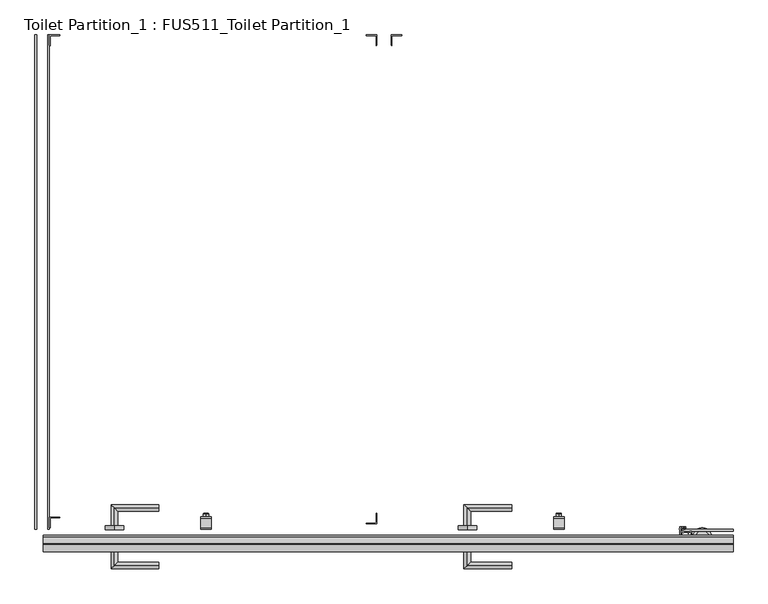
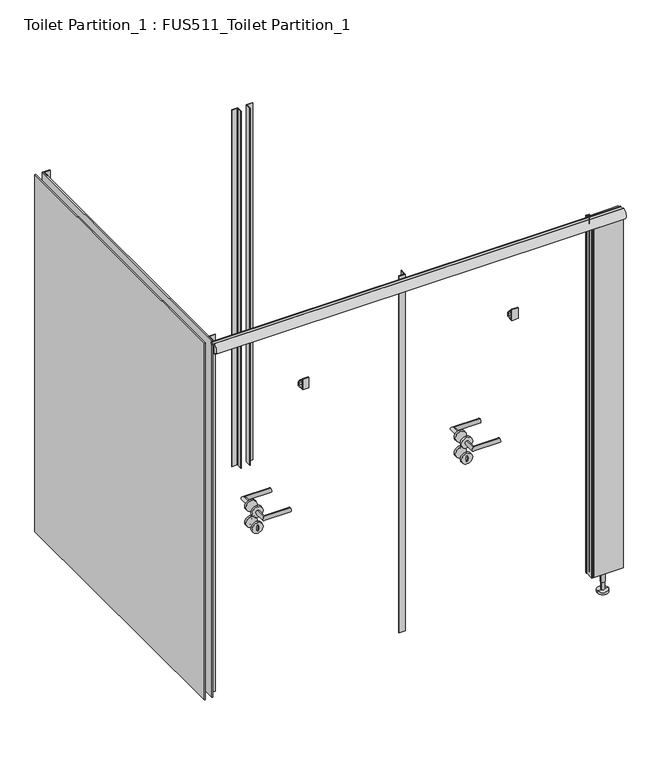
"""IFC4 building model written with IfcOpenShell, lengths in millimetres: furniture geometry, Toilet Partition_1 : FUS511_Toilet Partition_1."""

from ifc_helpers import new_model, si_unit, point, frame, frame_2d, origin, place, context, project, spatial, polyline, circle_curve, ellipse_curve, trimmed, segment, composite_curve, outline, extrude, source, transform, mapped, element, save
from ifc_brep_helpers import plane_surface, cylinder_surface, revolved_surface, extruded_surface, advanced_brep


def toilet_partition_1_fus511_toilet_partition_1_3647186f(model_context):
    return source(origin(), model_context, "Body", "SolidModel", [
        extrude(outline(polyline([(346.5617082, 503.4888254), (346.5617082, 497.0402783), (344.1649522, 497.0402783), (344.1649522, 497.8847941), (345.5746219, 497.8847941), (345.5746219, 501.5146528), (337.5048438, 501.5146528), (341.5634705, 497.0112968), (340.4236814, 497.0112968), (336.3650548, 501.5146528), (332.7425001, 501.5146528), (332.7425001, 454.1345106), (330.7683275, 454.1345106), (330.7683275, 497.4270801), (329.456802, 495.1554513), (328.3170129, 495.1554513), (330.7683275, 499.4012527), (330.7683275, 503.4888254), (346.5617082, 503.4888254)])), frame((0.0, 0.0, 100.0), z_axis=(0.0, 0.0, 1.0), x_axis=(1.0, 0.0, 0.0)), (0.0, 0.0, 1.0), 1800.0),
        extrude(outline(composite_curve([segment(trimmed(circle_curve(frame_2d((341.357373, 496.004016)), 0.789669), [point((341.357373, 495.214347))], [point((340.5677039, 496.004016))], False, "CARTESIAN"), True, "CONTINUOUS"), segment(polyline([(340.5677039, 496.004016), (340.5677039, 496.8402783), (341.715535, 496.8402783)]), True, "CONTINUOUS"), segment(trimmed(circle_curve(frame_2d((341.0726269, 497.4916495)), 0.9152132), [point((341.715535, 496.8402783))], [point((341.665841, 498.1885801))], True, "CARTESIAN"), True, "CONTINUOUS"), segment(trimmed(circle_curve(frame_2d((341.9239046, 498.4917631)), 0.3981417), [point((341.665841, 498.1885801))], [point((341.7737026, 498.8604854))], False, "CARTESIAN"), True, "CONTINUOUS"), segment(trimmed(circle_curve(frame_2d((342.8695936, 496.1702449)), 2.9048875), [point((341.7737026, 498.8604854))], [point((343.9414711, 498.870143))], False, "CARTESIAN"), True, "CONTINUOUS"), segment(trimmed(circle_curve(frame_2d((343.7877156, 498.4828563)), 0.4166915), [point((343.9414711, 498.870143))], [point((344.0660464, 498.1727534))], False, "CARTESIAN"), True, "CONTINUOUS"), segment(trimmed(circle_curve(frame_2d((344.6773667, 497.4916495)), 0.9152132), [point((344.0660464, 498.1727534))], [point((344.0344586, 496.8402783))], True, "CARTESIAN"), True, "CONTINUOUS"), segment(polyline([(344.0344586, 496.8402783), (345.1822897, 496.8402783), (345.1822897, 496.004016)]), True, "CONTINUOUS"), segment(trimmed(circle_curve(frame_2d((344.3926207, 496.004016)), 0.789669), [point((345.1822897, 496.004016))], [point((344.3926207, 495.214347))], False, "CARTESIAN"), True, "CONTINUOUS"), segment(polyline([(344.3926207, 495.214347), (341.357373, 495.214347)]), True, "CONTINUOUS")], self_intersect=False)), frame((0.0, 0.0, 100.0), z_axis=(0.0, 0.0, 1.0), x_axis=(1.0, 0.0, 0.0)), (0.0, 0.0, 1.0), 1800.0),
        advanced_brep(
        [(409.5372607, 474.714347, 104.1461397), (409.5372607, 474.714347, 101.0217555), (378.2934188, 474.714347, 101.0217555), (378.2934188, 474.714347, 104.1461397), (419.9518747, 474.714347, 0.0), (393.9153398, 474.714347, 0.0), (367.8788048, 474.714347, 0.0), (419.9518747, 474.714347, 10.414614), (367.8788048, 474.714347, 10.414614), (401.7263002, 474.714347, 10.414614), (386.1043793, 474.714347, 10.414614), (401.7263002, 474.714347, 52.0730698), (386.1043793, 474.714347, 52.0730698), (404.3299537, 474.714347, 52.0730698), (383.5007258, 474.714347, 52.0730698), (404.3299537, 474.714347, 101.0217555), (383.5007258, 474.714347, 101.0217555), (411.6201835, 474.714347, 104.1461397), (376.210496, 474.714347, 104.1461397), (411.6201835, 474.714347, 110.394908), (376.210496, 474.714347, 110.394908), (393.9153398, 474.714347, 110.394908)],
        [
            (0, 1),
            (1, 2, circle_curve(frame((393.9153398, 474.714347, 101.0217555), z_axis=(0.0, 0.0, 1.0), x_axis=(-1.0, 0.0, 0.0)), 15.6219209)),
            (2, 3),
            (3, 0, circle_curve(frame((393.9153398, 474.714347, 104.1461397), z_axis=(0.0, 0.0, -1.0), x_axis=(-1.0, 0.0, 0.0)), 15.6219209)),
            (2, 1, circle_curve(frame((393.9153398, 474.714347, 101.0217555), z_axis=(0.0, 0.0, 1.0), x_axis=(-1.0, 0.0, 0.0)), 15.6219209)),
            (0, 3, circle_curve(frame((393.9153398, 474.714347, 104.1461397), z_axis=(0.0, 0.0, -1.0), x_axis=(-1.0, 0.0, 0.0)), 15.6219209)),
            (4, 5),
            (5, 6),
            (6, 4, circle_curve(frame((393.9153398, 474.714347, 0.0), z_axis=(0.0, 0.0, -1.0), x_axis=(-1.0, 0.0, 0.0)), 26.0365349)),
            (4, 6, circle_curve(frame((393.9153398, 474.714347, 0.0), z_axis=(0.0, 0.0, -1.0), x_axis=(-1.0, 0.0, 0.0)), 26.0365349)),
            (7, 4),
            (6, 8),
            (8, 7, circle_curve(frame((393.9153398, 474.714347, 10.414614), z_axis=(0.0, 0.0, -1.0), x_axis=(-1.0, 0.0, 0.0)), 26.0365349)),
            (7, 8, circle_curve(frame((393.9153398, 474.714347, 10.414614), z_axis=(0.0, 0.0, -1.0), x_axis=(-1.0, 0.0, 0.0)), 26.0365349)),
            (9, 7),
            (8, 10),
            (10, 9, circle_curve(frame((393.9153398, 474.714347, 10.414614), z_axis=(0.0, 0.0, -1.0), x_axis=(-1.0, 0.0, 0.0)), 7.8109605)),
            (9, 10, circle_curve(frame((393.9153398, 474.714347, 10.414614), z_axis=(0.0, 0.0, -1.0), x_axis=(-1.0, 0.0, 0.0)), 7.8109605)),
            (11, 9),
            (10, 12),
            (12, 11, circle_curve(frame((393.9153398, 474.714347, 52.0730698), z_axis=(0.0, 0.0, -1.0), x_axis=(-1.0, 0.0, 0.0)), 7.8109605)),
            (11, 12, circle_curve(frame((393.9153398, 474.714347, 52.0730698), z_axis=(0.0, 0.0, -1.0), x_axis=(-1.0, 0.0, 0.0)), 7.8109605)),
            (13, 11),
            (12, 14),
            (14, 13, circle_curve(frame((393.9153398, 474.714347, 52.0730698), z_axis=(0.0, 0.0, -1.0), x_axis=(-1.0, 0.0, 0.0)), 10.414614)),
            (13, 14, circle_curve(frame((393.9153398, 474.714347, 52.0730698), z_axis=(0.0, 0.0, -1.0), x_axis=(-1.0, 0.0, 0.0)), 10.414614)),
            (15, 13),
            (14, 16),
            (16, 15, circle_curve(frame((393.9153398, 474.714347, 101.0217555), z_axis=(0.0, 0.0, -1.0), x_axis=(-1.0, 0.0, 0.0)), 10.414614)),
            (15, 16, circle_curve(frame((393.9153398, 474.714347, 101.0217555), z_axis=(0.0, 0.0, -1.0), x_axis=(-1.0, 0.0, 0.0)), 10.414614)),
            (1, 15),
            (16, 2),
            (17, 0),
            (3, 18),
            (18, 17, circle_curve(frame((393.9153398, 474.714347, 104.1461397), z_axis=(0.0, 0.0, -1.0), x_axis=(-1.0, 0.0, 0.0)), 17.7048437)),
            (17, 18, circle_curve(frame((393.9153398, 474.714347, 104.1461397), z_axis=(0.0, 0.0, -1.0), x_axis=(-1.0, 0.0, 0.0)), 17.7048437)),
            (19, 17),
            (18, 20),
            (20, 19, circle_curve(frame((393.9153398, 474.714347, 110.394908), z_axis=(0.0, 0.0, -1.0), x_axis=(-1.0, 0.0, 0.0)), 17.7048437)),
            (19, 20, circle_curve(frame((393.9153398, 474.714347, 110.394908), z_axis=(0.0, 0.0, -1.0), x_axis=(-1.0, 0.0, 0.0)), 17.7048437)),
            (21, 19),
            (20, 21),
        ],
        [
            cylinder_surface(frame((393.9153398, 474.714347, 190.0), z_axis=(0.0, 0.0, 1.0), x_axis=(-1.0, 0.0, 0.0)), 15.6219209),
            plane_surface(frame((393.9153398, 474.714347, 0.0), z_axis=(0.0, 0.0, -1.0), x_axis=(-1.0, 0.0, 0.0))),
            cylinder_surface(frame((393.9153398, 474.714347, 190.0), z_axis=(0.0, 0.0, 1.0), x_axis=(-1.0, 0.0, 0.0)), 26.0365349),
            plane_surface(frame((393.9153398, 474.714347, 10.414614), z_axis=(0.0, 0.0, 1.0), x_axis=(-1.0, 0.0, 0.0))),
            cylinder_surface(frame((393.9153398, 474.714347, 190.0), z_axis=(0.0, 0.0, 1.0), x_axis=(-1.0, 0.0, 0.0)), 7.8109605),
            plane_surface(frame((393.9153398, 474.714347, 52.0730698), z_axis=(0.0, 0.0, -1.0), x_axis=(-1.0, 0.0, 0.0))),
            cylinder_surface(frame((393.9153398, 474.714347, 190.0), z_axis=(0.0, 0.0, 1.0), x_axis=(-1.0, 0.0, 0.0)), 10.414614),
            plane_surface(frame((393.9153398, 474.714347, 101.0217555), z_axis=(0.0, 0.0, -1.0), x_axis=(-1.0, 0.0, 0.0))),
            plane_surface(frame((393.9153398, 474.714347, 104.1461397), z_axis=(0.0, 0.0, -1.0), x_axis=(-1.0, 0.0, 0.0))),
            cylinder_surface(frame((393.9153398, 474.714347, 190.0), z_axis=(0.0, 0.0, 1.0), x_axis=(-1.0, 0.0, 0.0)), 17.7048437),
            plane_surface(frame((393.9153398, 474.714347, 110.394908), z_axis=(0.0, 0.0, 1.0), x_axis=(-1.0, 0.0, 0.0))),
        ],
        [
            (0, [[1, 2, 3, 4]]),
            (0, [[-3, 5, -1, 6]]),
            (1, [[7, 8, 9]]),
            (1, [[-8, -7, 10]]),
            (2, [[11, -9, 12, 13]]),
            (2, [[-12, -10, -11, 14]]),
            (3, [[15, -13, 16, 17]]),
            (3, [[-16, -14, -15, 18]]),
            (4, [[19, -17, 20, 21]]),
            (4, [[-20, -18, -19, 22]]),
            (5, [[23, -21, 24, 25]]),
            (5, [[-24, -22, -23, 26]]),
            (6, [[27, -25, 28, 29]]),
            (6, [[-28, -26, -27, 30]]),
            (7, [[31, -29, 32, -2]]),
            (7, [[-32, -30, -31, -5]]),
            (8, [[33, -4, 34, 35]]),
            (8, [[-34, -6, -33, 36]]),
            (9, [[37, -35, 38, 39]]),
            (9, [[-38, -36, -37, 40]]),
            (10, [[41, -39, 42]]),
            (10, [[-42, -40, -41]]),
        ],
    ),
        extrude(outline(composite_curve([segment(polyline([(363.6512518, 489.5206414), (363.6512518, 459.9080525), (358.7158203, 459.9080525), (358.7158203, 460.8951388), (354.7674751, 460.8951388), (354.7674751, 459.9080525), (341.1950386, 459.9080525)]), True, "CONTINUOUS"), segment(trimmed(circle_curve(frame_2d((340.948267, 460.8637947)), 0.9870863), [point((341.1950386, 459.9080525))], [point((340.7014954, 459.9080525))], True, "CARTESIAN"), True, "CONTINUOUS"), segment(polyline([(340.7014954, 459.9080525), (336.0128355, 459.9080525), (336.0128355, 454.9726211), (335.0257492, 454.9726211)]), True, "CONTINUOUS"), segment(trimmed(circle_curve(frame_2d((335.0257492, 455.9597074)), 0.9870863), [point((335.0257492, 454.9726211))], [point((334.0386629, 455.9597074))], False, "CARTESIAN"), True, "CONTINUOUS"), segment(polyline([(334.0386629, 455.9597074), (334.0386629, 493.4689866)]), True, "CONTINUOUS"), segment(trimmed(circle_curve(frame_2d((335.0257492, 493.4689866)), 0.9870863), [point((334.0386629, 493.4689866))], [point((335.0257492, 494.4560729))], False, "CARTESIAN"), True, "CONTINUOUS"), segment(polyline([(335.0257492, 494.4560729), (336.0128355, 494.4560729), (336.0128355, 489.5206414), (340.7014954, 489.5206414)]), True, "CONTINUOUS"), segment(trimmed(circle_curve(frame_2d((340.948267, 488.5648992)), 0.9870863), [point((340.7014954, 489.5206414))], [point((341.1950386, 489.5206414))], True, "CARTESIAN"), True, "CONTINUOUS"), segment(polyline([(341.1950386, 489.5206414), (354.7674751, 488.5335551), (358.7158203, 488.5335551), (358.7158203, 489.5206414), (363.6512518, 489.5206414)]), True, "CONTINUOUS")], self_intersect=False), holes=[polyline([(360.6899929, 486.5593825), (355.7545614, 486.5593825), (355.7545614, 481.623951), (352.7933025, 481.623951), (352.7933025, 486.5593825), (345.8836985, 486.5593825), (345.8836985, 482.1174942), (344.403069, 482.1174942), (344.403069, 486.5593825), (342.675668, 486.5593825), (342.675668, 484.5852099), (338.7273228, 484.5852099), (338.7273228, 486.5593825), (336.9999218, 486.5593825), (336.9999218, 462.8693114), (338.7273228, 462.8693114), (338.7273228, 464.843484), (342.675668, 464.843484), (342.675668, 462.8693114), (344.403069, 462.8693114), (344.403069, 467.3111998), (345.8836985, 467.3111998), (345.8836985, 462.8693114), (352.7933025, 462.8693114), (352.7933025, 467.8047429), (355.7545614, 467.8047429), (355.7545614, 462.8693114), (360.6899929, 462.8693114), (360.6899929, 486.5593825)])]), frame((0.0, 0.0, 100.0), z_axis=(0.0, 0.0, 1.0), x_axis=(1.0, 0.0, 0.0)), (0.0, 0.0, 1.0), 1800.0),
        extrude(outline(polyline([(481.0128355, 454.214347), (336.0128355, 454.214347), (336.0128355, 459.214347), (481.0128355, 459.214347), (481.0128355, 454.214347)])), frame((0.0, 0.0, 100.0), z_axis=(0.0, 0.0, 1.0), x_axis=(1.0, 0.0, 0.0)), (0.0, 0.0, 1.0), 1800.0),
        extrude(outline(polyline([(481.0128355, 490.214347), (336.0128355, 490.214347), (336.0128355, 495.214347), (481.0128355, 495.214347), (481.0128355, 490.214347)])), frame((0.0, 0.0, 100.0), z_axis=(0.0, 0.0, 1.0), x_axis=(1.0, 0.0, 0.0)), (0.0, 0.0, 1.0), 1800.0),
        extrude(outline(composite_curve([segment(trimmed(circle_curve(frame_2d((-1451.3856706, 1892.2118377)), 1.0008364), [point((-1451.3856706, 1893.2126742))], [point((-1452.386507, 1892.2118377))], True, "CARTESIAN"), True, "CONTINUOUS"), segment(polyline([(-1452.386507, 1892.2118377), (-1452.386507, 1865.1892547), (-1453.3873434, 1865.1892547)]), True, "CONTINUOUS"), segment(trimmed(circle_curve(frame_2d((-1453.3873434, 1866.1900911)), 1.0008364), [point((-1453.3873434, 1865.1892547))], [point((-1454.3881798, 1866.1900911))], False, "CARTESIAN"), True, "CONTINUOUS"), segment(polyline([(-1454.3881798, 1866.1900911), (-1454.3881798, 1895.214347), (-1425.3639239, 1895.214347)]), True, "CONTINUOUS"), segment(trimmed(circle_curve(frame_2d((-1425.3639239, 1894.2135106)), 1.0008364), [point((-1425.3639239, 1895.214347))], [point((-1424.3630875, 1894.2135106))], False, "CARTESIAN"), True, "CONTINUOUS"), segment(polyline([(-1424.3630875, 1894.2135106), (-1424.3630875, 1893.2126742), (-1451.3856706, 1893.2126742)]), True, "CONTINUOUS")], self_intersect=False)), frame((0.0, 0.0, 100.0), z_axis=(0.0, 0.0, 1.0), x_axis=(1.0, 0.0, 0.0)), (0.0, 0.0, 1.0), 1800.0),
        extrude(outline(composite_curve([segment(trimmed(circle_curve(frame_2d((-1451.3856706, 527.0159753)), 1.0008364), [point((-1451.3856706, 528.0168117))], [point((-1452.386507, 527.0159753))], True, "CARTESIAN"), True, "CONTINUOUS"), segment(polyline([(-1452.386507, 527.0159753), (-1452.386507, 499.9933923), (-1453.3873434, 499.9933923)]), True, "CONTINUOUS"), segment(trimmed(circle_curve(frame_2d((-1453.3873434, 500.9942287)), 1.0008364), [point((-1453.3873434, 499.9933923))], [point((-1454.3881798, 500.9942287))], False, "CARTESIAN"), True, "CONTINUOUS"), segment(polyline([(-1454.3881798, 500.9942287), (-1454.3881798, 530.0184846), (-1425.3639239, 530.0184846)]), True, "CONTINUOUS"), segment(trimmed(circle_curve(frame_2d((-1425.3639239, 529.0176481)), 1.0008364), [point((-1425.3639239, 530.0184846))], [point((-1424.3630875, 529.0176481))], False, "CARTESIAN"), True, "CONTINUOUS"), segment(polyline([(-1424.3630875, 529.0176481), (-1424.3630875, 528.0168117), (-1451.3856706, 528.0168117)]), True, "CONTINUOUS")], self_intersect=False)), frame((0.0, 0.0, 100.0), z_axis=(0.0, 0.0, 1.0), x_axis=(1.0, 0.0, 0.0)), (0.0, 0.0, 1.0), 1800.0),
        extrude(outline(polyline([(-1454.3881798, 495.214347), (-1459.3881798, 495.214347), (-1459.3881798, 1895.214347), (-1454.3881798, 1895.214347), (-1454.3881798, 495.214347)])), frame((0.0, 0.0, 100.0), z_axis=(0.0, 0.0, 1.0), x_axis=(1.0, 0.0, 0.0)), (0.0, 0.0, 1.0), 1800.0),
        extrude(outline(polyline([(-1490.3881798, 495.214347), (-1495.3881798, 495.214347), (-1495.3881798, 1895.214347), (-1490.3881798, 1895.214347), (-1490.3881798, 495.214347)])), frame((0.0, 0.0, 100.0), z_axis=(0.0, 0.0, 1.0), x_axis=(1.0, 0.0, 0.0)), (0.0, 0.0, 1.0), 1800.0),
        advanced_brep(
        [(-271.279512, 505.214347, 893.5), (-271.279512, 505.214347, 946.5), (-271.279512, 505.214347, 934.6347495), (-271.279512, 505.214347, 904.6347495), (-271.279512, 495.214347, 893.5), (-271.279512, 495.214347, 946.5), (-271.279512, 499.9019579, 904.6347495), (-271.279512, 499.9019579, 934.6347495)],
        [
            (0, 1, circle_curve(frame((-271.279512, 505.214347, 920.0), z_axis=(0.0, 1.0, 0.0), x_axis=(0.0, 0.0, 1.0)), 26.5)),
            (1, 0, circle_curve(frame((-271.279512, 505.214347, 920.0), z_axis=(0.0, 1.0, 0.0), x_axis=(0.0, 0.0, 1.0)), 26.5)),
            (2, 3, ellipse_curve(frame((-271.279512, 505.214347, 919.6347495), z_axis=(0.0, -1.0, 0.0), x_axis=(0.0, 0.0, 1.0)), 15.0, 5.0)),
            (3, 2, ellipse_curve(frame((-271.279512, 505.214347, 919.6347495), z_axis=(0.0, -1.0, 0.0), x_axis=(0.0, 0.0, 1.0)), 15.0, 5.0)),
            (4, 5, circle_curve(frame((-271.279512, 495.214347, 920.0), z_axis=(0.0, -1.0, 0.0), x_axis=(0.0, 0.0, 1.0)), 26.5)),
            (5, 4, circle_curve(frame((-271.279512, 495.214347, 920.0), z_axis=(0.0, -1.0, 0.0), x_axis=(0.0, 0.0, 1.0)), 26.5)),
            (0, 4),
            (5, 1),
            (6, 7, ellipse_curve(frame((-271.279512, 499.9019579, 919.6347495), z_axis=(0.0, 1.0, 0.0), x_axis=(0.0, 0.0, 1.0)), 15.0, 5.0)),
            (7, 6, ellipse_curve(frame((-271.279512, 499.9019579, 919.6347495), z_axis=(0.0, 1.0, 0.0), x_axis=(0.0, 0.0, 1.0)), 15.0, 5.0)),
            (6, 3),
            (2, 7),
        ],
        [
            plane_surface(frame((-271.279512, 505.214347, 946.5), z_axis=(0.0, 1.0, 0.0), x_axis=(1.0, 0.0, 0.0))),
            plane_surface(frame((-271.279512, 495.214347, 946.5), z_axis=(0.0, -1.0, 0.0), x_axis=(-1.0, 0.0, 0.0))),
            cylinder_surface(frame((-271.279512, 495.214347, 920.0), z_axis=(0.0, 1.0, 0.0), x_axis=(0.0, 0.0, 1.0)), 26.5),
            plane_surface(frame((-271.279512, 499.9019579, 934.6347495), z_axis=(0.0, 1.0, 0.0), x_axis=(-1.0, 0.0, 0.0))),
            extruded_surface(trimmed(ellipse_curve(frame((-271.279512, 499.9019579, 919.6347495), z_axis=(0.0, 1.0, 0.0), x_axis=(0.0, 0.0, 1.0)), 15.0, 5.0), [point((-271.279512, 499.9019579, 904.6347495))], [point((-271.279512, 499.9019579, 934.6347495))], True, "CARTESIAN"), (0.0, -5.312388999999996, 0.0), 5.312388999999996),
            extruded_surface(trimmed(ellipse_curve(frame((-271.279512, 499.9019579, 919.6347495), z_axis=(0.0, 1.0, 0.0), x_axis=(0.0, 0.0, 1.0)), 15.0, 5.0), [point((-271.279512, 499.9019579, 934.6347495))], [point((-271.279512, 499.9019579, 904.6347495))], True, "CARTESIAN"), (0.0, -5.312388999999996, 0.0), 5.312388999999996),
        ],
        [
            (0, [[1, 2], [3, 4]]),
            (1, [[5, 6]]),
            (2, [[-1, 7, -6, 8]]),
            (2, [[-2, -8, -5, -7]]),
            (3, [[9, 10]]),
            (4, [[-9, 11, -3, 12]]),
            (5, [[-10, -12, -4, -11]]),
        ],
    ),
        advanced_brep(
        [(-271.279512, 505.214347, 990.5), (-271.279512, 505.214347, 1009.5), (-271.279512, 555.714347, 990.5), (-271.279512, 555.714347, 1009.5), (-145.779512, 555.714347, 990.5), (-145.779512, 555.714347, 1009.5)],
        [
            (0, 1, circle_curve(frame((-271.279512, 505.214347, 1000.0), z_axis=(0.0, -1.0, 0.0), x_axis=(0.0, 0.0, 1.0)), 9.5)),
            (1, 0, circle_curve(frame((-271.279512, 505.214347, 1000.0), z_axis=(0.0, -1.0, 0.0), x_axis=(0.0, 0.0, 1.0)), 9.5)),
            (0, 2),
            (2, 3, ellipse_curve(frame((-271.279512, 555.714347, 1000.0), z_axis=(-0.7071067811865486, -0.7071067811865465, 0.0), x_axis=(0.7071067811865465, -0.7071067811865485, 0.0)), 13.4350288, 9.5)),
            (3, 1),
            (3, 2, ellipse_curve(frame((-271.279512, 555.714347, 1000.0), z_axis=(-0.7071067811865486, -0.7071067811865465, 0.0), x_axis=(0.7071067811865465, -0.7071067811865485, 0.0)), 13.4350288, 9.5)),
            (4, 5, circle_curve(frame((-145.779512, 555.714347, 1000.0), z_axis=(1.0, 0.0, 0.0), x_axis=(0.0, 0.0, 1.0)), 9.5)),
            (5, 4, circle_curve(frame((-145.779512, 555.714347, 1000.0), z_axis=(1.0, 0.0, 0.0), x_axis=(0.0, 0.0, 1.0)), 9.5)),
            (2, 4),
            (5, 3),
        ],
        [
            plane_surface(frame((-280.779512, 505.214347, 1000.0), z_axis=(0.0, -1.0, 0.0), x_axis=(0.0, 0.0, 1.0))),
            cylinder_surface(frame((-271.279512, 505.214347, 1000.0), z_axis=(0.0, -1.0, 0.0), x_axis=(0.0, 0.0, 1.0)), 9.5),
            plane_surface(frame((-145.779512, 565.214347, 1000.0), z_axis=(1.0, 0.0, 0.0), x_axis=(0.0, 0.0, 1.0))),
            cylinder_surface(frame((-280.779512, 555.714347, 1000.0), z_axis=(-1.0, 0.0, 0.0), x_axis=(0.0, 0.0, 1.0)), 9.5),
        ],
        [
            (0, [[1, 2]]),
            (1, [[-1, 3, 4, 5]]),
            (1, [[-2, -5, 6, -3]]),
            (2, [[7, 8]]),
            (3, [[-4, 9, -8, 10]]),
            (3, [[-6, -10, -7, -9]]),
        ],
    ),
        extrude(outline(composite_curve([segment(trimmed(circle_curve(frame_2d((1000.0, -271.279512)), 26.5), [point((973.5, -271.279512))], [point((1026.5, -271.279512))], False, "CARTESIAN"), True, "CONTINUOUS"), segment(trimmed(circle_curve(frame_2d((1000.0, -271.279512)), 26.5), [point((1026.5, -271.279512))], [point((973.5, -271.279512))], False, "CARTESIAN"), True, "CONTINUOUS")], self_intersect=False)), frame((0.0, 495.214347, 0.0), z_axis=(0.0, 1.0, 0.0), x_axis=(0.0, 0.0, 1.0)), (0.0, 0.0, 1.0), 10.0),
        advanced_brep(
        [(-1270.2108466, 505.214347, 893.5), (-1270.2108466, 505.214347, 946.5), (-1270.2108466, 505.214347, 934.6347495), (-1270.2108466, 505.214347, 904.6347495), (-1270.2108466, 495.214347, 893.5), (-1270.2108466, 495.214347, 946.5), (-1270.2108466, 499.9019579, 904.6347495), (-1270.2108466, 499.9019579, 934.6347495)],
        [
            (0, 1, circle_curve(frame((-1270.2108466, 505.214347, 920.0), z_axis=(0.0, 1.0, 0.0), x_axis=(0.0, 0.0, 1.0)), 26.5)),
            (1, 0, circle_curve(frame((-1270.2108466, 505.214347, 920.0), z_axis=(0.0, 1.0, 0.0), x_axis=(0.0, 0.0, 1.0)), 26.5)),
            (2, 3, ellipse_curve(frame((-1270.2108466, 505.214347, 919.6347495), z_axis=(0.0, -1.0, 0.0), x_axis=(0.0, 0.0, 1.0)), 15.0, 5.0)),
            (3, 2, ellipse_curve(frame((-1270.2108466, 505.214347, 919.6347495), z_axis=(0.0, -1.0, 0.0), x_axis=(0.0, 0.0, 1.0)), 15.0, 5.0)),
            (4, 5, circle_curve(frame((-1270.2108466, 495.214347, 920.0), z_axis=(0.0, -1.0, 0.0), x_axis=(0.0, 0.0, 1.0)), 26.5)),
            (5, 4, circle_curve(frame((-1270.2108466, 495.214347, 920.0), z_axis=(0.0, -1.0, 0.0), x_axis=(0.0, 0.0, 1.0)), 26.5)),
            (0, 4),
            (5, 1),
            (6, 7, ellipse_curve(frame((-1270.2108466, 499.9019579, 919.6347495), z_axis=(0.0, 1.0, 0.0), x_axis=(0.0, 0.0, 1.0)), 15.0, 5.0)),
            (7, 6, ellipse_curve(frame((-1270.2108466, 499.9019579, 919.6347495), z_axis=(0.0, 1.0, 0.0), x_axis=(0.0, 0.0, 1.0)), 15.0, 5.0)),
            (6, 3),
            (2, 7),
        ],
        [
            plane_surface(frame((-1270.2108466, 505.214347, 946.5), z_axis=(0.0, 1.0, 0.0), x_axis=(1.0, 0.0, 0.0))),
            plane_surface(frame((-1270.2108466, 495.214347, 946.5), z_axis=(0.0, -1.0, 0.0), x_axis=(-1.0, 0.0, 0.0))),
            cylinder_surface(frame((-1270.2108466, 495.214347, 920.0), z_axis=(0.0, 1.0, 0.0), x_axis=(0.0, 0.0, 1.0)), 26.5),
            plane_surface(frame((-1270.2108466, 499.9019579, 934.6347495), z_axis=(0.0, 1.0, 0.0), x_axis=(-1.0, 0.0, 0.0))),
            extruded_surface(trimmed(ellipse_curve(frame((-1270.2108466, 499.9019579, 919.6347495), z_axis=(0.0, 1.0, 0.0), x_axis=(0.0, 0.0, 1.0)), 15.0, 5.0), [point((-1270.2108466, 499.9019579, 904.6347495))], [point((-1270.2108466, 499.9019579, 934.6347495))], True, "CARTESIAN"), (0.0, -5.312388999999996, 0.0), 5.312388999999996),
            extruded_surface(trimmed(ellipse_curve(frame((-1270.2108466, 499.9019579, 919.6347495), z_axis=(0.0, 1.0, 0.0), x_axis=(0.0, 0.0, 1.0)), 15.0, 5.0), [point((-1270.2108466, 499.9019579, 934.6347495))], [point((-1270.2108466, 499.9019579, 904.6347495))], True, "CARTESIAN"), (0.0, -5.312388999999996, 0.0), 5.312388999999996),
        ],
        [
            (0, [[1, 2], [3, 4]]),
            (1, [[5, 6]]),
            (2, [[-1, 7, -6, 8]]),
            (2, [[-2, -8, -5, -7]]),
            (3, [[9, 10]]),
            (4, [[-9, 11, -3, 12]]),
            (5, [[-10, -12, -4, -11]]),
        ],
    ),
        advanced_brep(
        [(-1270.2108466, 505.214347, 990.5), (-1270.2108466, 505.214347, 1009.5), (-1270.2108466, 555.714347, 990.5), (-1270.2108466, 555.714347, 1009.5), (-1144.7108466, 555.714347, 990.5), (-1144.7108466, 555.714347, 1009.5)],
        [
            (0, 1, circle_curve(frame((-1270.2108466, 505.214347, 1000.0), z_axis=(0.0, -1.0, 0.0), x_axis=(0.0, 0.0, 1.0)), 9.5)),
            (1, 0, circle_curve(frame((-1270.2108466, 505.214347, 1000.0), z_axis=(0.0, -1.0, 0.0), x_axis=(0.0, 0.0, 1.0)), 9.5)),
            (0, 2),
            (2, 3, ellipse_curve(frame((-1270.2108466, 555.714347, 1000.0), z_axis=(-0.7071067811865486, -0.7071067811865465, 0.0), x_axis=(0.7071067811865465, -0.7071067811865485, 0.0)), 13.4350288, 9.5)),
            (3, 1),
            (3, 2, ellipse_curve(frame((-1270.2108466, 555.714347, 1000.0), z_axis=(-0.7071067811865486, -0.7071067811865465, 0.0), x_axis=(0.7071067811865465, -0.7071067811865485, 0.0)), 13.4350288, 9.5)),
            (4, 5, circle_curve(frame((-1144.7108466, 555.714347, 1000.0), z_axis=(1.0, 0.0, 0.0), x_axis=(0.0, 0.0, 1.0)), 9.5)),
            (5, 4, circle_curve(frame((-1144.7108466, 555.714347, 1000.0), z_axis=(1.0, 0.0, 0.0), x_axis=(0.0, 0.0, 1.0)), 9.5)),
            (2, 4),
            (5, 3),
        ],
        [
            plane_surface(frame((-1279.7108466, 505.214347, 1000.0), z_axis=(0.0, -1.0, 0.0), x_axis=(0.0, 0.0, 1.0))),
            cylinder_surface(frame((-1270.2108466, 505.214347, 1000.0), z_axis=(0.0, -1.0, 0.0), x_axis=(0.0, 0.0, 1.0)), 9.5),
            plane_surface(frame((-1144.7108466, 565.214347, 1000.0), z_axis=(1.0, 0.0, 0.0), x_axis=(0.0, 0.0, 1.0))),
            cylinder_surface(frame((-1279.7108466, 555.714347, 1000.0), z_axis=(-1.0, 0.0, 0.0), x_axis=(0.0, 0.0, 1.0)), 9.5),
        ],
        [
            (0, [[1, 2]]),
            (1, [[-1, 3, 4, 5]]),
            (1, [[-2, -5, 6, -3]]),
            (2, [[7, 8]]),
            (3, [[-4, 9, -8, 10]]),
            (3, [[-6, -10, -7, -9]]),
        ],
    ),
        extrude(outline(composite_curve([segment(trimmed(circle_curve(frame_2d((1000.0, -1270.2108466)), 26.5), [point((973.5, -1270.2108466))], [point((1026.5, -1270.2108466))], False, "CARTESIAN"), True, "CONTINUOUS"), segment(trimmed(circle_curve(frame_2d((1000.0, -1270.2108466)), 26.5), [point((1026.5, -1270.2108466))], [point((973.5, -1270.2108466))], False, "CARTESIAN"), True, "CONTINUOUS")], self_intersect=False)), frame((0.0, 495.214347, 0.0), z_axis=(0.0, 1.0, 0.0), x_axis=(0.0, 0.0, 1.0)), (0.0, 0.0, 1.0), 10.0),
        advanced_brep(
        [(-271.279512, 444.214347, 893.5), (-271.279512, 444.214347, 946.5), (-271.279512, 444.214347, 934.6347495), (-271.279512, 444.214347, 904.6347495), (-271.279512, 454.214347, 893.5), (-271.279512, 454.214347, 946.5), (-271.279512, 449.526736, 904.6347495), (-271.279512, 449.526736, 934.6347495)],
        [
            (0, 1, circle_curve(frame((-271.279512, 444.214347, 920.0), z_axis=(0.0, -1.0, 0.0), x_axis=(0.0, 0.0, 1.0)), 26.5)),
            (1, 0, circle_curve(frame((-271.279512, 444.214347, 920.0), z_axis=(0.0, -1.0, 0.0), x_axis=(0.0, 0.0, 1.0)), 26.5)),
            (2, 3, ellipse_curve(frame((-271.279512, 444.214347, 919.6347495), z_axis=(0.0, 1.0, 0.0), x_axis=(0.0, 0.0, 1.0)), 15.0, 5.0)),
            (3, 2, ellipse_curve(frame((-271.279512, 444.214347, 919.6347495), z_axis=(0.0, 1.0, 0.0), x_axis=(0.0, 0.0, 1.0)), 15.0, 5.0)),
            (4, 5, circle_curve(frame((-271.279512, 454.214347, 920.0), z_axis=(0.0, 1.0, 0.0), x_axis=(0.0, 0.0, 1.0)), 26.5)),
            (5, 4, circle_curve(frame((-271.279512, 454.214347, 920.0), z_axis=(0.0, 1.0, 0.0), x_axis=(0.0, 0.0, 1.0)), 26.5)),
            (1, 5),
            (4, 0),
            (6, 7, ellipse_curve(frame((-271.279512, 449.526736, 919.6347495), z_axis=(0.0, -1.0, 0.0), x_axis=(0.0, 0.0, 1.0)), 15.0, 5.0)),
            (7, 6, ellipse_curve(frame((-271.279512, 449.526736, 919.6347495), z_axis=(0.0, -1.0, 0.0), x_axis=(0.0, 0.0, 1.0)), 15.0, 5.0)),
            (7, 2),
            (3, 6),
        ],
        [
            plane_surface(frame((-271.279512, 444.214347, 946.5), z_axis=(0.0, -1.0, 0.0), x_axis=(1.0, 0.0, 0.0))),
            plane_surface(frame((-271.279512, 454.214347, 946.5), z_axis=(0.0, 1.0, 0.0), x_axis=(-1.0, 0.0, 0.0))),
            cylinder_surface(frame((-271.279512, 454.214347, 920.0), z_axis=(0.0, -1.0, 0.0), x_axis=(0.0, 0.0, 1.0)), 26.5),
            plane_surface(frame((-271.279512, 449.526736, 934.6347495), z_axis=(0.0, -1.0, 0.0), x_axis=(-1.0, 0.0, 0.0))),
            extruded_surface(trimmed(ellipse_curve(frame((-271.279512, 454.8391251, 919.6347495), z_axis=(0.0, 1.0, 0.0), x_axis=(0.0, 0.0, 1.0)), 15.0, 5.0), [point((-271.279512, 454.8391251, 904.6347495))], [point((-271.279512, 454.8391251, 934.6347495))], True, "CARTESIAN"), (0.0, -5.312389099999962, 0.0), 5.312389099999962),
            extruded_surface(trimmed(ellipse_curve(frame((-271.279512, 454.8391251, 919.6347495), z_axis=(0.0, 1.0, 0.0), x_axis=(0.0, 0.0, 1.0)), 15.0, 5.0), [point((-271.279512, 454.8391251, 934.6347495))], [point((-271.279512, 454.8391251, 904.6347495))], True, "CARTESIAN"), (0.0, -5.312389099999962, 0.0), 5.312389099999962),
        ],
        [
            (0, [[1, 2], [3, 4]]),
            (1, [[5, 6]]),
            (2, [[7, -5, 8, -2]]),
            (2, [[-8, -6, -7, -1]]),
            (3, [[9, 10]]),
            (4, [[11, -4, 12, -10]]),
            (5, [[-12, -3, -11, -9]]),
        ],
    ),
        advanced_brep(
        [(-271.279512, 444.214347, 990.5), (-271.279512, 444.214347, 1009.5), (-271.279512, 393.714347, 1009.5), (-271.279512, 393.714347, 990.5), (-145.779512, 393.714347, 990.5), (-145.779512, 393.714347, 1009.5)],
        [
            (0, 1, circle_curve(frame((-271.279512, 444.214347, 1000.0), z_axis=(0.0, 1.0, 0.0), x_axis=(0.0, 0.0, 1.0)), 9.5)),
            (1, 0, circle_curve(frame((-271.279512, 444.214347, 1000.0), z_axis=(0.0, 1.0, 0.0), x_axis=(0.0, 0.0, 1.0)), 9.5)),
            (1, 2),
            (2, 3, ellipse_curve(frame((-271.279512, 393.714347, 1000.0), z_axis=(-0.7071067811865486, 0.7071067811865465, 0.0), x_axis=(0.7071067811865465, 0.7071067811865485, 0.0)), 13.4350288, 9.5)),
            (3, 0),
            (3, 2, ellipse_curve(frame((-271.279512, 393.714347, 1000.0), z_axis=(-0.7071067811865486, 0.7071067811865465, 0.0), x_axis=(0.7071067811865465, 0.7071067811865485, 0.0)), 13.4350288, 9.5)),
            (4, 5, circle_curve(frame((-145.779512, 393.714347, 1000.0), z_axis=(1.0, 0.0, 0.0), x_axis=(0.0, 0.0, 1.0)), 9.5)),
            (5, 4, circle_curve(frame((-145.779512, 393.714347, 1000.0), z_axis=(1.0, 0.0, 0.0), x_axis=(0.0, 0.0, 1.0)), 9.5)),
            (2, 5),
            (4, 3),
        ],
        [
            plane_surface(frame((-280.779512, 444.214347, 1000.0), z_axis=(0.0, 1.0, 0.0), x_axis=(0.0, 0.0, 1.0))),
            cylinder_surface(frame((-271.279512, 444.214347, 1000.0), z_axis=(0.0, 1.0, 0.0), x_axis=(0.0, 0.0, 1.0)), 9.5),
            plane_surface(frame((-145.779512, 384.214347, 1000.0), z_axis=(1.0, 0.0, 0.0), x_axis=(0.0, 0.0, 1.0))),
            cylinder_surface(frame((-280.779512, 393.714347, 1000.0), z_axis=(-1.0, 0.0, 0.0), x_axis=(0.0, 0.0, 1.0)), 9.5),
        ],
        [
            (0, [[1, 2]]),
            (1, [[3, 4, 5, -2]]),
            (1, [[-5, 6, -3, -1]]),
            (2, [[7, 8]]),
            (3, [[9, -7, 10, -4]]),
            (3, [[-10, -8, -9, -6]]),
        ],
    ),
        extrude(outline(composite_curve([segment(trimmed(circle_curve(frame_2d((1000.0, -271.279512)), 26.5), [point((973.5, -271.279512))], [point((1026.5, -271.279512))], False, "CARTESIAN"), True, "CONTINUOUS"), segment(trimmed(circle_curve(frame_2d((1000.0, -271.279512)), 26.5), [point((1026.5, -271.279512))], [point((973.5, -271.279512))], False, "CARTESIAN"), True, "CONTINUOUS")], self_intersect=False)), frame((0.0, 444.214347, 0.0), z_axis=(0.0, 1.0, 0.0), x_axis=(0.0, 0.0, 1.0)), (0.0, 0.0, 1.0), 10.0),
        advanced_brep(
        [(-1270.2108466, 444.214347, 893.5), (-1270.2108466, 444.214347, 946.5), (-1270.2108466, 444.214347, 934.6347495), (-1270.2108466, 444.214347, 904.6347495), (-1270.2108466, 454.214347, 893.5), (-1270.2108466, 454.214347, 946.5), (-1270.2108466, 449.526736, 904.6347495), (-1270.2108466, 449.526736, 934.6347495)],
        [
            (0, 1, circle_curve(frame((-1270.2108466, 444.214347, 920.0), z_axis=(0.0, -1.0, 0.0), x_axis=(0.0, 0.0, 1.0)), 26.5)),
            (1, 0, circle_curve(frame((-1270.2108466, 444.214347, 920.0), z_axis=(0.0, -1.0, 0.0), x_axis=(0.0, 0.0, 1.0)), 26.5)),
            (2, 3, ellipse_curve(frame((-1270.2108466, 444.214347, 919.6347495), z_axis=(0.0, 1.0, 0.0), x_axis=(0.0, 0.0, 1.0)), 15.0, 5.0)),
            (3, 2, ellipse_curve(frame((-1270.2108466, 444.214347, 919.6347495), z_axis=(0.0, 1.0, 0.0), x_axis=(0.0, 0.0, 1.0)), 15.0, 5.0)),
            (4, 5, circle_curve(frame((-1270.2108466, 454.214347, 920.0), z_axis=(0.0, 1.0, 0.0), x_axis=(0.0, 0.0, 1.0)), 26.5)),
            (5, 4, circle_curve(frame((-1270.2108466, 454.214347, 920.0), z_axis=(0.0, 1.0, 0.0), x_axis=(0.0, 0.0, 1.0)), 26.5)),
            (1, 5),
            (4, 0),
            (6, 7, ellipse_curve(frame((-1270.2108466, 449.526736, 919.6347495), z_axis=(0.0, -1.0, 0.0), x_axis=(0.0, 0.0, 1.0)), 15.0, 5.0)),
            (7, 6, ellipse_curve(frame((-1270.2108466, 449.526736, 919.6347495), z_axis=(0.0, -1.0, 0.0), x_axis=(0.0, 0.0, 1.0)), 15.0, 5.0)),
            (7, 2),
            (3, 6),
        ],
        [
            plane_surface(frame((-1270.2108466, 444.214347, 946.5), z_axis=(0.0, -1.0, 0.0), x_axis=(1.0, 0.0, 0.0))),
            plane_surface(frame((-1270.2108466, 454.214347, 946.5), z_axis=(0.0, 1.0, 0.0), x_axis=(-1.0, 0.0, 0.0))),
            cylinder_surface(frame((-1270.2108466, 454.214347, 920.0), z_axis=(0.0, -1.0, 0.0), x_axis=(0.0, 0.0, 1.0)), 26.5),
            plane_surface(frame((-1270.2108466, 449.526736, 934.6347495), z_axis=(0.0, -1.0, 0.0), x_axis=(-1.0, 0.0, 0.0))),
            extruded_surface(trimmed(ellipse_curve(frame((-1270.2108466, 454.8391251, 919.6347495), z_axis=(0.0, 1.0, 0.0), x_axis=(0.0, 0.0, 1.0)), 15.0, 5.0), [point((-1270.2108466, 454.8391251, 904.6347495))], [point((-1270.2108466, 454.8391251, 934.6347495))], True, "CARTESIAN"), (0.0, -5.312389099999962, 0.0), 5.312389099999962),
            extruded_surface(trimmed(ellipse_curve(frame((-1270.2108466, 454.8391251, 919.6347495), z_axis=(0.0, 1.0, 0.0), x_axis=(0.0, 0.0, 1.0)), 15.0, 5.0), [point((-1270.2108466, 454.8391251, 934.6347495))], [point((-1270.2108466, 454.8391251, 904.6347495))], True, "CARTESIAN"), (0.0, -5.312389099999962, 0.0), 5.312389099999962),
        ],
        [
            (0, [[1, 2], [3, 4]]),
            (1, [[5, 6]]),
            (2, [[7, -5, 8, -2]]),
            (2, [[-8, -6, -7, -1]]),
            (3, [[9, 10]]),
            (4, [[11, -4, 12, -10]]),
            (5, [[-12, -3, -11, -9]]),
        ],
    ),
        advanced_brep(
        [(-1270.2108466, 444.214347, 990.5), (-1270.2108466, 444.214347, 1009.5), (-1270.2108466, 393.714347, 1009.5), (-1270.2108466, 393.714347, 990.5), (-1144.7108466, 393.714347, 990.5), (-1144.7108466, 393.714347, 1009.5)],
        [
            (0, 1, circle_curve(frame((-1270.2108466, 444.214347, 1000.0), z_axis=(0.0, 1.0, 0.0), x_axis=(0.0, 0.0, 1.0)), 9.5)),
            (1, 0, circle_curve(frame((-1270.2108466, 444.214347, 1000.0), z_axis=(0.0, 1.0, 0.0), x_axis=(0.0, 0.0, 1.0)), 9.5)),
            (1, 2),
            (2, 3, ellipse_curve(frame((-1270.2108466, 393.714347, 1000.0), z_axis=(-0.7071067811865486, 0.7071067811865465, 0.0), x_axis=(0.7071067811865465, 0.7071067811865485, 0.0)), 13.4350288, 9.5)),
            (3, 0),
            (3, 2, ellipse_curve(frame((-1270.2108466, 393.714347, 1000.0), z_axis=(-0.7071067811865486, 0.7071067811865465, 0.0), x_axis=(0.7071067811865465, 0.7071067811865485, 0.0)), 13.4350288, 9.5)),
            (4, 5, circle_curve(frame((-1144.7108466, 393.714347, 1000.0), z_axis=(1.0, 0.0, 0.0), x_axis=(0.0, 0.0, 1.0)), 9.5)),
            (5, 4, circle_curve(frame((-1144.7108466, 393.714347, 1000.0), z_axis=(1.0, 0.0, 0.0), x_axis=(0.0, 0.0, 1.0)), 9.5)),
            (2, 5),
            (4, 3),
        ],
        [
            plane_surface(frame((-1279.7108466, 444.214347, 1000.0), z_axis=(0.0, 1.0, 0.0), x_axis=(0.0, 0.0, 1.0))),
            cylinder_surface(frame((-1270.2108466, 444.214347, 1000.0), z_axis=(0.0, 1.0, 0.0), x_axis=(0.0, 0.0, 1.0)), 9.5),
            plane_surface(frame((-1144.7108466, 384.214347, 1000.0), z_axis=(1.0, 0.0, 0.0), x_axis=(0.0, 0.0, 1.0))),
            cylinder_surface(frame((-1279.7108466, 393.714347, 1000.0), z_axis=(-1.0, 0.0, 0.0), x_axis=(0.0, 0.0, 1.0)), 9.5),
        ],
        [
            (0, [[1, 2]]),
            (1, [[3, 4, 5, -2]]),
            (1, [[-5, 6, -3, -1]]),
            (2, [[7, 8]]),
            (3, [[9, -7, 10, -4]]),
            (3, [[-10, -8, -9, -6]]),
        ],
    ),
        extrude(outline(composite_curve([segment(trimmed(circle_curve(frame_2d((1000.0, -1270.2108466)), 26.5), [point((973.5, -1270.2108466))], [point((1026.5, -1270.2108466))], False, "CARTESIAN"), True, "CONTINUOUS"), segment(trimmed(circle_curve(frame_2d((1000.0, -1270.2108466)), 26.5), [point((1026.5, -1270.2108466))], [point((973.5, -1270.2108466))], False, "CARTESIAN"), True, "CONTINUOUS")], self_intersect=False)), frame((0.0, 444.214347, 0.0), z_axis=(0.0, 1.0, 0.0), x_axis=(0.0, 0.0, 1.0)), (0.0, 0.0, 1.0), 10.0),
        extrude(outline(composite_curve([segment(trimmed(circle_curve(frame_2d((458.4868618, 1888.0268612)), 26.5042707), [point((454.214347, 1861.869224))], [point((453.0212869, 1913.9614685))], False, "CARTESIAN"), True, "CONTINUOUS"), segment(trimmed(circle_curve(frame_2d((453.1556919, 1912.91138)), 1.058655), [point((453.0212869, 1913.9614685))], [point((454.214347, 1912.91138))], False, "CARTESIAN"), True, "CONTINUOUS"), segment(polyline([(454.214347, 1912.91138), (454.214347, 1909.5278954), (474.6592543, 1909.5278954)]), True, "CONTINUOUS"), segment(trimmed(circle_curve(frame_2d((474.2293597, 1904.6828737)), 4.8640564), [point((474.6592543, 1909.5278954))], [point((479.0927404, 1904.7639477))], False, "CARTESIAN"), True, "CONTINUOUS"), segment(trimmed(circle_curve(frame_2d((474.2293597, 1904.8450217)), 4.8640564), [point((479.0927404, 1904.7639477))], [point((473.7994652, 1900.0))], False, "CARTESIAN"), True, "CONTINUOUS"), segment(polyline([(473.7994652, 1900.0), (454.214347, 1900.0), (454.214347, 1861.869224)]), True, "CONTINUOUS")], self_intersect=False), holes=[composite_curve([segment(polyline([(473.939812, 1907.9461271), (455.8017383, 1907.9399126), (455.8017383, 1901.5879827), (473.9398142, 1901.5817682)]), True, "CONTINUOUS"), segment(trimmed(circle_curve(frame_2d((473.9325063, 1904.7639477)), 3.1821878), [point((473.9398142, 1901.5817682))], [point((473.939812, 1907.9461271))], True, "CARTESIAN"), True, "CONTINUOUS")], self_intersect=False), composite_curve([segment(trimmed(circle_curve(frame_2d((457.6658618, 1888.0268612)), 24.6245189), [point((452.6263644, 1912.1301887))], [point((452.6263644, 1863.9235337))], True, "CARTESIAN"), True, "CONTINUOUS"), segment(polyline([(452.6263644, 1863.9235337), (452.6263644, 1912.1301887)]), True, "CONTINUOUS")], self_intersect=False)]), frame((-1471.8881798, 0.0, 0.0), z_axis=(1.0, 0.0, 0.0), x_axis=(0.0, 1.0, 0.0)), (0.0, 0.0, 1.0), 1953.0),
        extrude(outline(composite_curve([segment(polyline([(499.2367016, 1553.2961991), (499.2367016, 1504.0), (527.3931841, 1504.0), (527.3931841, 1516.0894186)]), True, "CONTINUOUS"), segment(trimmed(circle_curve(frame_2d((531.4155388, 1516.0894186)), 4.0223546), [point((527.3931841, 1516.0894186))], [point((531.4155388, 1520.1117732))], False, "CARTESIAN"), True, "CONTINUOUS"), segment(polyline([(531.4155388, 1520.1117732), (531.4155388, 1500.0), (499.2367016, 1500.0), (495.214347, 1500.0), (495.214347, 1553.2961991), (499.2367016, 1553.2961991)]), True, "CONTINUOUS")], self_intersect=False)), frame((-1026.1694992, 0.0, 0.0), z_axis=(1.0, 0.0, 0.0), x_axis=(0.0, 1.0, 0.0)), (0.0, 0.0, 1.0), 30.0),
        advanced_brep(
        [(-1011.1694992, 531.4155388, 1510.5586809), (-1011.1694992, 531.4155388, 1518.1005959), (-1011.1694992, 531.4155388, 1503.016766), (-1011.1694992, 541.4714254, 1506.033532), (-1011.1694992, 541.4714254, 1515.0838299), (-1011.1694992, 541.4714254, 1510.5586809), (-1011.1694992, 539.4602481, 1503.016766), (-1011.1694992, 539.4602481, 1518.1005959)],
        [
            (0, 1),
            (1, 2, circle_curve(frame((-1011.1694992, 531.4155388, 1510.5586809), z_axis=(0.0, -1.0, 0.0), x_axis=(0.0, 0.0, 1.0)), 7.541915)),
            (2, 0),
            (2, 1, circle_curve(frame((-1011.1694992, 531.4155388, 1510.5586809), z_axis=(0.0, -1.0, 0.0), x_axis=(0.0, 0.0, 1.0)), 7.541915)),
            (3, 4, circle_curve(frame((-1011.1694992, 541.4714254, 1510.5586809), z_axis=(0.0, 1.0, 0.0), x_axis=(0.0, 0.0, 1.0)), 4.525149)),
            (4, 5),
            (5, 3),
            (4, 3, circle_curve(frame((-1011.1694992, 541.4714254, 1510.5586809), z_axis=(0.0, 1.0, 0.0), x_axis=(0.0, 0.0, 1.0)), 4.525149)),
            (6, 7, circle_curve(frame((-1011.1694992, 539.4602481, 1510.5586809), z_axis=(0.0, 1.0, 0.0), x_axis=(0.0, 0.0, 1.0)), 7.541915)),
            (7, 4, circle_curve(frame((-1011.1694992, 538.111954, 1515.0229578), z_axis=(-1.0, 0.0, 0.0), x_axis=(0.0, 0.0, -1.0)), 3.3600228)),
            (3, 6, circle_curve(frame((-1011.1694992, 538.111954, 1506.0944041), z_axis=(-1.0, 0.0, 0.0), x_axis=(0.0, 0.0, 1.0)), 3.3600228)),
            (7, 6, circle_curve(frame((-1011.1694992, 539.4602481, 1510.5586809), z_axis=(0.0, 1.0, 0.0), x_axis=(0.0, 0.0, 1.0)), 7.541915)),
            (1, 7),
            (6, 2),
        ],
        [
            plane_surface(frame((-1011.1694992, 531.4155388, 1510.5586809), z_axis=(0.0, -1.0, 0.0), x_axis=(0.0, 0.0, 1.0))),
            plane_surface(frame((-1011.1694992, 541.4714254, 1510.5586809), z_axis=(0.0, 1.0, 0.0), x_axis=(0.0, 0.0, 1.0))),
            revolved_surface(trimmed(ellipse_curve(frame((-1011.1694992, 538.111954, 1515.0229578), z_axis=(1.0, 0.0, 0.0), x_axis=(0.0, 0.0, -1.0)), 3.3600228, 3.3600228), [point((-1011.1694992, 541.4714254, 1515.0838299))], [point((-1011.1694992, 539.4602481, 1518.1005959))], True, "CARTESIAN"), (-1011.1694992, 521.4714254, 1510.5586809), (0.0, -1.0, 0.0)),
            cylinder_surface(frame((-1011.1694992, 521.4714254, 1510.5586809), z_axis=(0.0, -1.0, 0.0), x_axis=(0.0, 0.0, 1.0)), 7.541915),
        ],
        [
            (0, [[1, 2, 3]]),
            (0, [[-3, 4, -1]]),
            (1, [[5, 6, 7]]),
            (1, [[8, -7, -6]]),
            (2, [[9, 10, -5, 11]]),
            (2, [[12, -11, -8, -10]]),
            (3, [[-2, 13, -9, 14]]),
            (3, [[-4, -14, -12, -13]]),
        ],
    ),
        extrude(outline(composite_curve([segment(polyline([(499.2367016, 1553.2961991), (499.2367016, 1504.0), (527.3931841, 1504.0), (527.3931841, 1516.0894186)]), True, "CONTINUOUS"), segment(trimmed(circle_curve(frame_2d((531.4155388, 1516.0894186)), 4.0223546), [point((527.3931841, 1516.0894186))], [point((531.4155388, 1520.1117732))], False, "CARTESIAN"), True, "CONTINUOUS"), segment(polyline([(531.4155388, 1520.1117732), (531.4155388, 1500.0), (499.2367016, 1500.0), (495.214347, 1500.0), (495.214347, 1553.2961991), (499.2367016, 1553.2961991)]), True, "CONTINUOUS")], self_intersect=False)), frame((-27.2381646, 0.0, 0.0), z_axis=(1.0, 0.0, 0.0), x_axis=(0.0, 1.0, 0.0)), (0.0, 0.0, 1.0), 30.0),
        advanced_brep(
        [(-12.2381646, 531.4155388, 1510.5586809), (-12.2381646, 531.4155388, 1518.1005959), (-12.2381646, 531.4155388, 1503.016766), (-12.2381646, 541.4714254, 1506.033532), (-12.2381646, 541.4714254, 1515.0838299), (-12.2381646, 541.4714254, 1510.5586809), (-12.2381646, 539.4602481, 1503.016766), (-12.2381646, 539.4602481, 1518.1005959)],
        [
            (0, 1),
            (1, 2, circle_curve(frame((-12.2381646, 531.4155388, 1510.5586809), z_axis=(0.0, -1.0, 0.0), x_axis=(0.0, 0.0, 1.0)), 7.541915)),
            (2, 0),
            (2, 1, circle_curve(frame((-12.2381646, 531.4155388, 1510.5586809), z_axis=(0.0, -1.0, 0.0), x_axis=(0.0, 0.0, 1.0)), 7.541915)),
            (3, 4, circle_curve(frame((-12.2381646, 541.4714254, 1510.5586809), z_axis=(0.0, 1.0, 0.0), x_axis=(0.0, 0.0, 1.0)), 4.525149)),
            (4, 5),
            (5, 3),
            (4, 3, circle_curve(frame((-12.2381646, 541.4714254, 1510.5586809), z_axis=(0.0, 1.0, 0.0), x_axis=(0.0, 0.0, 1.0)), 4.525149)),
            (6, 7, circle_curve(frame((-12.2381646, 539.4602481, 1510.5586809), z_axis=(0.0, 1.0, 0.0), x_axis=(0.0, 0.0, 1.0)), 7.541915)),
            (7, 4, circle_curve(frame((-12.2381646, 538.111954, 1515.0229578), z_axis=(-1.0, 0.0, 0.0), x_axis=(0.0, 0.0, -1.0)), 3.3600228)),
            (3, 6, circle_curve(frame((-12.2381646, 538.111954, 1506.0944041), z_axis=(-1.0, 0.0, 0.0), x_axis=(0.0, 0.0, 1.0)), 3.3600228)),
            (7, 6, circle_curve(frame((-12.2381646, 539.4602481, 1510.5586809), z_axis=(0.0, 1.0, 0.0), x_axis=(0.0, 0.0, 1.0)), 7.541915)),
            (1, 7),
            (6, 2),
        ],
        [
            plane_surface(frame((-12.2381646, 531.4155388, 1510.5586809), z_axis=(0.0, -1.0, 0.0), x_axis=(0.0, 0.0, 1.0))),
            plane_surface(frame((-12.2381646, 541.4714254, 1510.5586809), z_axis=(0.0, 1.0, 0.0), x_axis=(0.0, 0.0, 1.0))),
            revolved_surface(trimmed(ellipse_curve(frame((-12.2381646, 538.111954, 1515.0229578), z_axis=(1.0, 0.0, 0.0), x_axis=(0.0, 0.0, -1.0)), 3.3600228, 3.3600228), [point((-12.2381646, 541.4714254, 1515.0838299))], [point((-12.2381646, 539.4602481, 1518.1005959))], True, "CARTESIAN"), (-12.2381646, 521.4714254, 1510.5586809), (0.0, -1.0, 0.0)),
            cylinder_surface(frame((-12.2381646, 521.4714254, 1510.5586809), z_axis=(0.0, -1.0, 0.0), x_axis=(0.0, 0.0, 1.0)), 7.541915),
        ],
        [
            (0, [[1, 2, 3]]),
            (0, [[-3, 4, -1]]),
            (1, [[5, 6, 7]]),
            (1, [[8, -7, -6]]),
            (2, [[9, 10, -5, 11]]),
            (2, [[12, -11, -8, -10]]),
            (3, [[-2, 13, -9, 14]]),
            (3, [[-4, -14, -12, -13]]),
        ],
    ),
        extrude(outline(composite_curve([segment(polyline([(-530.6901814, 1893.2126742), (-557.7127644, 1893.2126742), (-557.7127644, 1894.2135106)]), True, "CONTINUOUS"), segment(trimmed(circle_curve(frame_2d((-556.711928, 1894.2135106)), 1.0008364), [point((-557.7127644, 1894.2135106))], [point((-556.711928, 1895.214347))], False, "CARTESIAN"), True, "CONTINUOUS"), segment(polyline([(-556.711928, 1895.214347), (-527.6876721, 1895.214347), (-527.6876721, 1866.1900911)]), True, "CONTINUOUS"), segment(trimmed(circle_curve(frame_2d((-528.6885085, 1866.1900911)), 1.0008364), [point((-527.6876721, 1866.1900911))], [point((-528.6885085, 1865.1892547))], False, "CARTESIAN"), True, "CONTINUOUS"), segment(polyline([(-528.6885085, 1865.1892547), (-529.689345, 1865.1892547), (-529.689345, 1892.2118377)]), True, "CONTINUOUS"), segment(trimmed(circle_curve(frame_2d((-530.6901814, 1892.2118377)), 1.0008364), [point((-529.689345, 1892.2118377))], [point((-530.6901814, 1893.2126742))], True, "CARTESIAN"), True, "CONTINUOUS")], self_intersect=False)), frame((0.0, 0.0, 100.0), z_axis=(0.0, 0.0, 1.0), x_axis=(1.0, 0.0, 0.0)), (0.0, 0.0, 1.0), 1800.0),
        extrude(outline(composite_curve([segment(trimmed(circle_curve(frame_2d((-483.6851629, 1892.2118377)), 1.0008364), [point((-483.6851629, 1893.2126742))], [point((-484.6859993, 1892.2118377))], True, "CARTESIAN"), True, "CONTINUOUS"), segment(polyline([(-484.6859993, 1892.2118377), (-484.6859993, 1865.1892547), (-485.6868357, 1865.1892547)]), True, "CONTINUOUS"), segment(trimmed(circle_curve(frame_2d((-485.6868357, 1866.1900911)), 1.0008364), [point((-485.6868357, 1865.1892547))], [point((-486.6876721, 1866.1900911))], False, "CARTESIAN"), True, "CONTINUOUS"), segment(polyline([(-486.6876721, 1866.1900911), (-486.6876721, 1895.214347), (-457.6634163, 1895.214347)]), True, "CONTINUOUS"), segment(trimmed(circle_curve(frame_2d((-457.6634163, 1894.2135106)), 1.0008364), [point((-457.6634163, 1895.214347))], [point((-456.6625798, 1894.2135106))], False, "CARTESIAN"), True, "CONTINUOUS"), segment(polyline([(-456.6625798, 1894.2135106), (-456.6625798, 1893.2126742), (-483.6851629, 1893.2126742)]), True, "CONTINUOUS")], self_intersect=False)), frame((0.0, 0.0, 100.0), z_axis=(0.0, 0.0, 1.0), x_axis=(1.0, 0.0, 0.0)), (0.0, 0.0, 1.0), 1800.0),
        extrude(outline(composite_curve([segment(trimmed(circle_curve(frame_2d((-530.6901814, 514.4572016)), 1.0008364), [point((-530.6901814, 513.4563652))], [point((-529.689345, 514.4572016))], True, "CARTESIAN"), True, "CONTINUOUS"), segment(polyline([(-529.689345, 514.4572016), (-529.689345, 541.4797847), (-528.6885085, 541.4797847)]), True, "CONTINUOUS"), segment(trimmed(circle_curve(frame_2d((-528.6885085, 540.4789483)), 1.0008364), [point((-528.6885085, 541.4797847))], [point((-527.6876721, 540.4789483))], False, "CARTESIAN"), True, "CONTINUOUS"), segment(polyline([(-527.6876721, 540.4789483), (-527.6876721, 511.4546924), (-556.711928, 511.4546924)]), True, "CONTINUOUS"), segment(trimmed(circle_curve(frame_2d((-556.711928, 512.4555288)), 1.0008364), [point((-556.711928, 511.4546924))], [point((-557.7127644, 512.4555288))], False, "CARTESIAN"), True, "CONTINUOUS"), segment(polyline([(-557.7127644, 512.4555288), (-557.7127644, 513.4563652), (-530.6901814, 513.4563652)]), True, "CONTINUOUS")], self_intersect=False)), frame((0.0, 0.0, 100.0), z_axis=(0.0, 0.0, 1.0), x_axis=(1.0, 0.0, 0.0)), (0.0, 0.0, 1.0), 1800.0),
    ])


if __name__ == "__main__":
    model = new_model("IFC4")
    model_context = context("Model", 3, world=origin())
    ifc_project = project(units=[si_unit("LENGTHUNIT", "METRE", prefix="MILLI")], contexts=[model_context])
    site = spatial("IfcSite", under=ifc_project)
    building = spatial("IfcBuilding", under=site)
    placement = place(None, origin())
    toilet_partition_1_fus511_toilet_partition_1_shape = toilet_partition_1_fus511_toilet_partition_1_3647186f(model_context)
    element("IfcFurniture", 1, ObjectType="Toilet Partition_1 : FUS511_Toilet Partition_1", at=placement, inside=building, context=model_context, shape_type="MappedRepresentation", body=[
        mapped(toilet_partition_1_fus511_toilet_partition_1_shape, transform((0.0, 0.0, 0.0), x_axis=(1.0, 0.0, 0.0), y_axis=(0.0, 1.0, 0.0), z_axis=(0.0, 0.0, 1.0))),
    ])
    save(model, "model.ifc")

# Revit data of these elements
# Type "Toilet Partition_1 : FUS511_Toilet Partition_1"
#   Created by = "Utku Can Kocadağ"
#   Controlled by = "Sefer Özdoğan"
#   Approved by = "Aydın Altınova"
#   Cubicle_Height = 1800 mm
#   Bot_Gap = 100 mm
#   Default Elevation = 0
# Element 1 (IfcFurniture, "Toilet Partition_1 : FUS511_Toilet Partition_1")
#   Materials on its faces: "Aln_Aluminum_02"
# Materials
#   "Aln_Aluminum_02": class "Generic", colour RGB 120 120 120, transparency 0, Cost = 0
